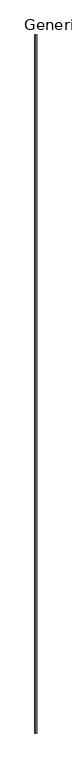
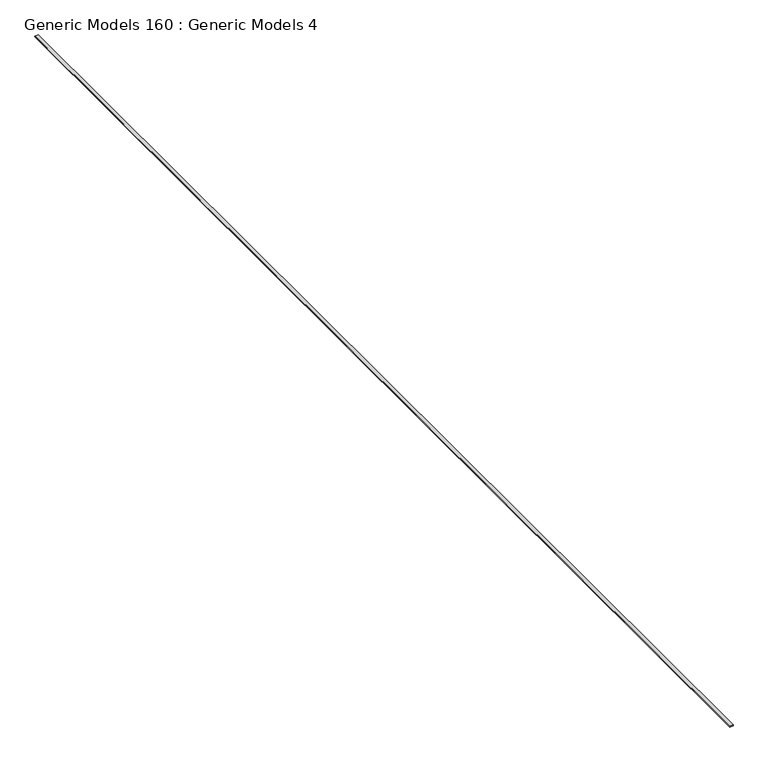
"""IFC4 building model written with IfcOpenShell, lengths in millimetres: proxy geometry, Generic Models 160 : Generic Models 4."""

from ifc_helpers import new_model, si_unit, point, frame, frame_2d, origin, place, context, project, spatial, polyline, circle_curve, trimmed, segment, composite_curve, outline, extrude, source, transform, mapped, element, save


def generic_models_160_generic_models_4_b938c61c(model_context):
    return source(origin(), model_context, "Body", "SweptSolid", [
        extrude(outline(composite_curve([segment(trimmed(circle_curve(frame_2d((122788.9609874, -10292.4988366)), 5.3394144), [point((122793.7234874, -10290.0847239))], [point((122784.1984874, -10290.0847239))], True, "CARTESIAN"), True, "CONTINUOUS"), segment(polyline([(122784.1984874, -10290.0847239), (122784.1984874, -10252.9339552), (122793.7234874, -10252.9339552), (122793.7234874, -10290.0847239)]), True, "CONTINUOUS")], self_intersect=False)), frame((0.0, -5493.3230338, 0.0), z_axis=(0.0, 1.0, 0.0), x_axis=(0.0, 0.0, 1.0)), (0.0, 0.0, 1.0), 12547.6),
    ])


if __name__ == "__main__":
    model = new_model("IFC4")
    model_context = context("Model", 3, world=origin())
    ifc_project = project(units=[si_unit("LENGTHUNIT", "METRE", prefix="MILLI")], contexts=[model_context])
    site = spatial("IfcSite", under=ifc_project)
    building = spatial("IfcBuilding", under=site)
    placement = place(None, origin())
    generic_models_160_generic_models_4_shape = generic_models_160_generic_models_4_b938c61c(model_context)
    element("IfcBuildingElementProxy", 1, Name="Generic Models 160 : Generic Models 4", ObjectType="Generic Models 160 : Generic Models 4", at=placement, inside=building, context=model_context, shape_type="MappedRepresentation", body=[
        mapped(generic_models_160_generic_models_4_shape, transform((0.0, 0.0, 0.0), x_axis=(1.0, 0.0, 0.0), y_axis=(0.0, 1.0, 0.0), z_axis=(0.0, 0.0, 1.0))),
    ])
    save(model, "model.ifc")

# Revit data of these elements
# Element 1 (IfcBuildingElementProxy, "Generic Models 160 : Generic Models 4")
#   Materials on its faces: "_MORTAR SETTING BED"
# Materials
#   "_MORTAR SETTING BED": class "Generic", colour RGB 191 191 191, transparency 0, Cost = 0
